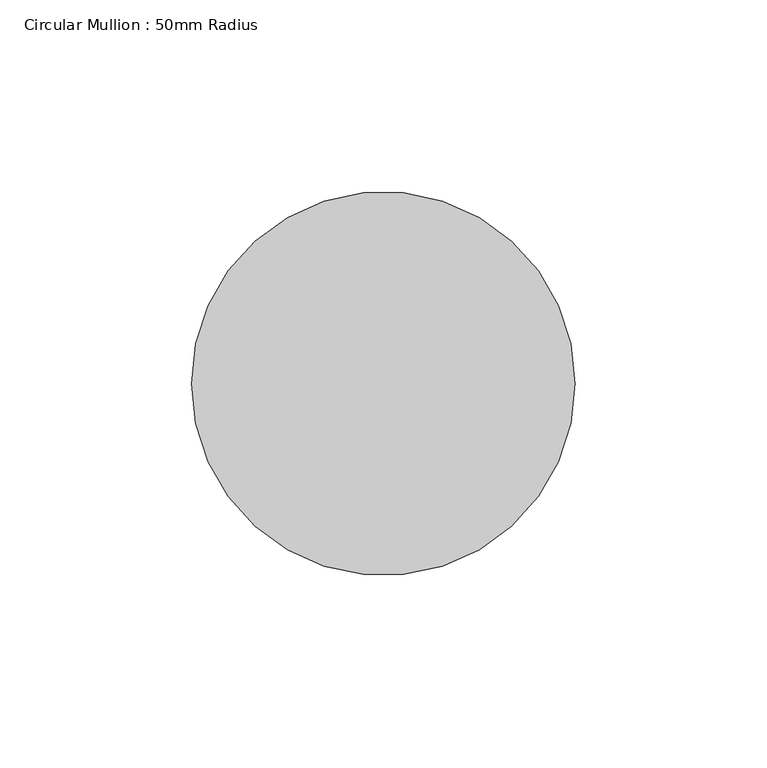
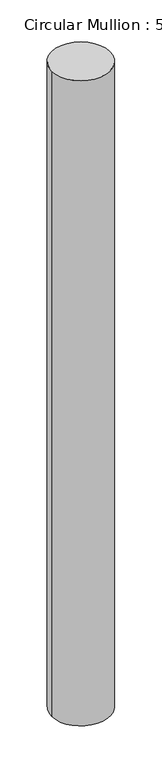
"""IFC4 building model written with IfcOpenShell, lengths in millimetres: member geometry, Circular Mullion : 50mm Radius."""

import ifcopenshell
import ifcopenshell.guid

model = None  # the IFC model being written
_history = None  # IfcOwnerHistory: only IFC2X3 demands one
_inside = {}  # id of a spatial element -> (the spatial element, [elements in it])
_under = {}  # id of a project, library or spatial element -> (it, [spatial elements below it])
_declared = {}  # id of a project -> (the project, [libraries it declares])
_typed = {}  # id of a type object -> (the type object, [elements of that type])
_made_of = {}  # id of a material, layer set ... -> (it, [elements and type objects made of it])


def new_model(schema):
    """Start an empty IFC model of exactly this schema.

    Asked for "IFC4X3", IfcOpenShell would pick the latest addendum, in which some entities
    have other attributes; the version numbers below select the first issue.
    IFC2X3 requires an IfcOwnerHistory on every rooted entity: one is made here for all.
    """
    global model, _history
    if schema == "IFC4X3":
        model = ifcopenshell.file(schema_version=(4, 3, 0, 0))
    else:
        model = ifcopenshell.file(schema=schema)
    _inside.clear()
    _under.clear()
    _declared.clear()
    _typed.clear()
    _made_of.clear()
    _history = None
    if model.schema == "IFC2X3":
        org = make("IfcOrganization", Name="unknown")
        user = make(
            "IfcPersonAndOrganization",
            ThePerson=make("IfcPerson", FamilyName="unknown"),
            TheOrganization=org,
        )
        app = make(
            "IfcApplication",
            ApplicationDeveloper=org,
            Version="unknown",
            ApplicationFullName="unknown",
            ApplicationIdentifier="unknown",
        )
        _history = make(
            "IfcOwnerHistory",
            OwningUser=user,
            OwningApplication=app,
            ChangeAction="ADDED",
            CreationDate=0,
        )
    return model


def make(cls, **values):
    """One entity of the class cls with the attributes given. An attribute that is None is left unset."""
    return model.create_entity(
        cls, **{name: value for name, value in values.items() if value is not None}
    )


def rooted(cls, **values):
    """An entity with a GlobalId (a new one), such as an element, a storey or a relation."""
    return make(cls, GlobalId=ifcopenshell.guid.new(), OwnerHistory=_history, **values)


def si_unit(unit_type, name, prefix=None):
    """IfcSIUnit, for example si_unit("LENGTHUNIT", "METRE", prefix="MILLI")."""
    return make("IfcSIUnit", UnitType=unit_type, Prefix=prefix, Name=name)


def assignment(units):
    """IfcUnitAssignment: the units of a project."""
    return None if units is None else make("IfcUnitAssignment", Units=units)


def point(xyz):
    """IfcCartesianPoint."""
    return None if xyz is None else make("IfcCartesianPoint", Coordinates=xyz)


def direction(xyz):
    """IfcDirection."""
    return None if xyz is None else make("IfcDirection", DirectionRatios=xyz)


def frame(location, z_axis=None, x_axis=None):
    """IfcAxis2Placement3D, a coordinate frame: its origin and axes. An axis left out is left unset."""
    return make(
        "IfcAxis2Placement3D",
        Location=point(location),
        Axis=direction(z_axis),
        RefDirection=direction(x_axis),
    )


def frame_2d(location, x_axis=None):
    """IfcAxis2Placement2D, a coordinate frame in the plane: its origin and x axis."""
    return make(
        "IfcAxis2Placement2D", Location=point(location), RefDirection=direction(x_axis)
    )


def origin():
    """The frame at (0, 0, 0) with its axes left unset."""
    return frame((0.0, 0.0, 0.0))


def origin_2d():
    """The frame at (0, 0) in the plane with its x axis left unset."""
    return frame_2d((0.0, 0.0))


def place(relative_to, where):
    """IfcLocalPlacement: puts the frame where relative to a parent placement (None: the world)."""
    return make(
        "IfcLocalPlacement", PlacementRelTo=relative_to, RelativePlacement=where
    )


def context(
    kind, dimensions, precision=None, world=None, true_north=None, identifier=None
):
    """IfcGeometricRepresentationContext, for example the 3D "Model" context."""
    return make(
        "IfcGeometricRepresentationContext",
        ContextIdentifier=identifier,
        ContextType=kind,
        CoordinateSpaceDimension=dimensions,
        Precision=precision,
        WorldCoordinateSystem=world,
        TrueNorth=true_north,
    )


def project(units=None, contexts=None):
    """IfcProject with its units and contexts."""
    return rooted(
        "IfcProject",
        Name="project",
        RepresentationContexts=contexts,
        UnitsInContext=assignment(units),
    )


def spatial(cls, under=None, at=None, **own):
    """A site, building, storey or space (cls), placed at a placement, below another one or the project."""
    s = rooted(cls, ObjectPlacement=at, **own)
    if under is not None:
        _under.setdefault(under.id(), (under, []))[1].append(s)
    return s


def circle_curve(where, radius):
    """IfcCircle in the frame where."""
    return make("IfcCircle", Position=where, Radius=radius)


def trimmed(basis, trim1, trim2, sense, master):
    """IfcTrimmedCurve: the piece of a basis curve between two trims."""
    return make(
        "IfcTrimmedCurve",
        BasisCurve=basis,
        Trim1=trim1,
        Trim2=trim2,
        SenseAgreement=sense,
        MasterRepresentation=master,
    )


def segment(curve, same_sense, transition):
    """IfcCompositeCurveSegment."""
    return make(
        "IfcCompositeCurveSegment",
        Transition=transition,
        SameSense=same_sense,
        ParentCurve=curve,
    )


def composite_curve(segments, self_intersect=None):
    """IfcCompositeCurve: segments joined end to end."""
    return make("IfcCompositeCurve", Segments=segments, SelfIntersect=self_intersect)


def outline(outer, holes=None, kind="AREA"):
    """IfcArbitraryClosedProfileDef: a profile drawn as a closed curve; with holes, ...WithVoids."""
    if holes is None:
        return make("IfcArbitraryClosedProfileDef", ProfileType=kind, OuterCurve=outer)
    return make(
        "IfcArbitraryProfileDefWithVoids",
        ProfileType=kind,
        OuterCurve=outer,
        InnerCurves=holes,
    )


def extrude(swept, where, along, depth):
    """IfcExtrudedAreaSolid: the profile swept, set in the frame where, extruded along a direction by depth."""
    return make(
        "IfcExtrudedAreaSolid",
        SweptArea=swept,
        Position=where,
        ExtrudedDirection=direction(along),
        Depth=depth,
    )


def shape(context_of_items, identifier, shape_type, items):
    """IfcShapeRepresentation: the items that make up one representation, for example the "Body"."""
    return make(
        "IfcShapeRepresentation",
        ContextOfItems=context_of_items,
        RepresentationIdentifier=identifier,
        RepresentationType=shape_type,
        Items=items,
    )


def source(mapping_origin, context_of_items, identifier, shape_type, items):
    """IfcRepresentationMap: a shape defined once, which mapped items show again and again."""
    return make(
        "IfcRepresentationMap",
        MappingOrigin=mapping_origin,
        MappedRepresentation=shape(context_of_items, identifier, shape_type, items),
    )


def transform(
    local_origin,
    x_axis=None,
    y_axis=None,
    z_axis=None,
    scale=None,
    scale2=None,
    scale3=None,
    uniform=True,
):
    """IfcCartesianTransformationOperator3D, or its non-uniform kind. x_axis, y_axis, z_axis: its Axis1, 2, 3."""
    if uniform:
        return make(
            "IfcCartesianTransformationOperator3D",
            Axis1=direction(x_axis),
            Axis2=direction(y_axis),
            LocalOrigin=point(local_origin),
            Scale=scale,
            Axis3=direction(z_axis),
        )
    return make(
        "IfcCartesianTransformationOperator3DnonUniform",
        Axis1=direction(x_axis),
        Axis2=direction(y_axis),
        LocalOrigin=point(local_origin),
        Scale=scale,
        Axis3=direction(z_axis),
        Scale2=scale2,
        Scale3=scale3,
    )


def mapped(mapping_source, mapping_target):
    """IfcMappedItem: shows the shape of a source again, moved by a transform."""
    return make(
        "IfcMappedItem", MappingSource=mapping_source, MappingTarget=mapping_target
    )


def made_of(thing, what):
    """Note that an element or type object is made of a material, layer set ...; save() writes the relation."""
    if what is not None:
        _made_of.setdefault(what.id(), (what, []))[1].append(thing)
    return thing


def element(
    cls,
    number,
    at=None,
    inside=None,
    cuts=None,
    type_object=None,
    material=None,
    context=None,
    identifier="Body",
    shape_type=None,
    held_by="IfcProductDefinitionShape",
    body=None,
    shapes=None,
    **own,
):
    """One element of the class cls, such as IfcWall. Its Tag is "e" and its number.

    at: its placement. inside: the storey or other place that contains it. cuts: it is an
    opening in that element (IfcRelVoidsElement). A single representation is given by context,
    identifier, shape_type and body (its items); several are given by shapes. held_by: the class
    of the entity that holds the representations. save() writes the other relations.
    """
    e = rooted(cls, Tag="e%d" % number, ObjectPlacement=at, **own)
    if body is not None:
        shapes = [shape(context, identifier, shape_type, body)]
    if shapes is not None:
        e.Representation = make(held_by, Representations=shapes)
    if inside is not None:
        _inside.setdefault(inside.id(), (inside, []))[1].append(e)
    if cuts is not None:
        rooted(
            "IfcRelVoidsElement", RelatingBuildingElement=cuts, RelatedOpeningElement=e
        )
    if type_object is not None:
        _typed.setdefault(type_object.id(), (type_object, []))[1].append(e)
    return made_of(e, material)


def aggregate(whole, parts):
    """IfcRelAggregates: a whole, such as a stair, and the parts it consists of."""
    return rooted("IfcRelAggregates", RelatingObject=whole, RelatedObjects=parts)


def save(model, path):
    """Write the relations noted so far, then the file.

    IfcRelAggregates (storeys below a building ...), IfcRelContainedInSpatialStructure (elements
    in a storey), IfcRelDefinesByType, IfcRelAssociatesMaterial and IfcRelDeclares: one each for
    every whole, place, type object, material and project.
    """
    for whole, parts in _under.values():
        aggregate(whole, parts)
    for where, things in _inside.values():
        rooted(
            "IfcRelContainedInSpatialStructure",
            RelatedElements=things,
            RelatingStructure=where,
        )
    for kind, things in _typed.values():
        rooted("IfcRelDefinesByType", RelatedObjects=things, RelatingType=kind)
    for what, things in _made_of.values():
        rooted("IfcRelAssociatesMaterial", RelatedObjects=things, RelatingMaterial=what)
    for by, libraries in _declared.values():
        rooted("IfcRelDeclares", RelatingContext=by, RelatedDefinitions=libraries)
    model.write(path)


def circular_mullion_50mm_radius_0d7448f9(model_context):
    return source(origin(), model_context, "Body", "SweptSolid", [
        extrude(outline(composite_curve([segment(trimmed(circle_curve(origin_2d(), 50.0), [point((50.0, 0.0))], [point((-50.0, 0.0))], False, "CARTESIAN"), True, "CONTINUOUS"), segment(trimmed(circle_curve(origin_2d(), 50.0), [point((-50.0, 0.0))], [point((50.0, 0.0))], False, "CARTESIAN"), True, "CONTINUOUS")], self_intersect=False)), frame((0.0, 0.0, -1166.7785492), z_axis=(0.0, 0.0, 1.0), x_axis=(1.0, 0.0, 0.0)), (0.0, 0.0, 1.0), 1166.7785492),
    ])


if __name__ == "__main__":
    model = new_model("IFC4")
    model_context = context("Model", 3, world=origin())
    ifc_project = project(units=[si_unit("LENGTHUNIT", "METRE", prefix="MILLI")], contexts=[model_context])
    site = spatial("IfcSite", under=ifc_project)
    building = spatial("IfcBuilding", under=site)
    placement = place(None, origin())
    circular_mullion_50mm_radius_shape = circular_mullion_50mm_radius_0d7448f9(model_context)
    element("IfcMember", 1, ObjectType="Circular Mullion : 50mm Radius", at=placement, inside=building, context=model_context, shape_type="MappedRepresentation", body=[
        mapped(circular_mullion_50mm_radius_shape, transform((0.0, 0.0, 0.0), x_axis=(1.0, 0.0, 0.0), y_axis=(0.0, 1.0, 0.0), z_axis=(0.0, 0.0, 1.0))),
    ])
    save(model, "model.ifc")

# Revit data of these elements
# Type "Circular Mullion : 50mm Radius"
#   built-in parameter 1007350 = 0.164042 (stored number, unit not read)
# Element 1 (IfcMember, "Circular Mullion : 50mm Radius")
#   Materials on its faces: "Aluminium"
# Materials
#   "Aluminium": class "Metal", colour RGB 247 247 247, transparency 0, Description = "Aluminium 6061", Cost = 0
